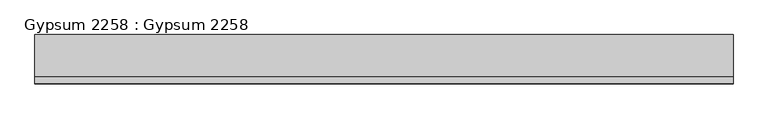
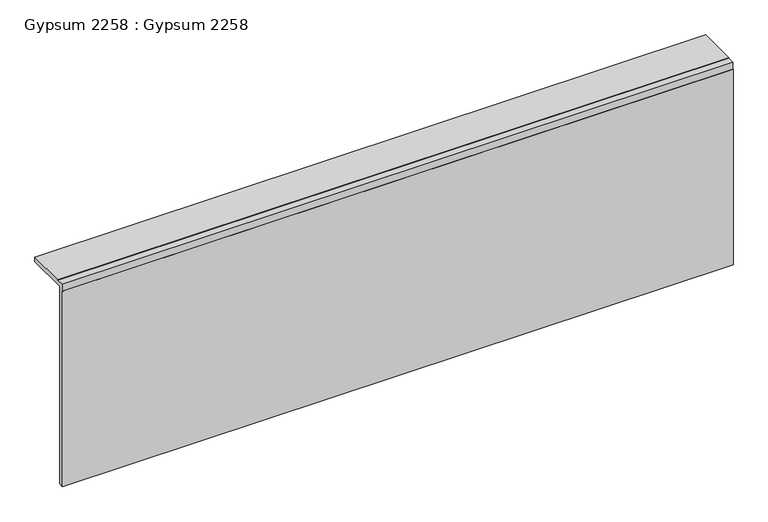
"""IFC4 building model written with IfcOpenShell, lengths in millimetres: proxy geometry, Gypsum 2258 : Gypsum 2258."""

from ifc_helpers import new_model, si_unit, frame, origin, place, context, project, spatial, polyline, outline, extrude, source, transform, mapped, element, save


def gypsum_2258_gypsum_2258_91d050d9(model_context):
    return source(origin(), model_context, "Body", "SweptSolid", [
        extrude(outline(polyline([(10263.7368438, 40772.8800973), (10265.0168438, 40772.8800973), (10265.0168438, 40794.0332812), (10286.1700277, 40794.0332812), (10286.1700277, 40795.3132812), (10405.3793386, 40795.3132812), (10405.3793386, 40779.84375), (10278.0250834, 40779.84375), (10278.0250834, 40157.1476563), (10263.7368438, 40157.1476563), (10263.7368438, 40772.8800973)])), frame((3694.2883192, 0.0, 0.0), z_axis=(1.0, 0.0, 0.0), x_axis=(0.0, 1.0, 0.0)), (0.0, 0.0, 1.0), 2000.0),
    ])


if __name__ == "__main__":
    model = new_model("IFC4")
    model_context = context("Model", 3, world=origin())
    ifc_project = project(units=[si_unit("LENGTHUNIT", "METRE", prefix="MILLI")], contexts=[model_context])
    site = spatial("IfcSite", under=ifc_project)
    building = spatial("IfcBuilding", under=site)
    placement = place(None, origin())
    gypsum_2258_gypsum_2258_shape = gypsum_2258_gypsum_2258_91d050d9(model_context)
    element("IfcBuildingElementProxy", 1, Name="Gypsum 2258 : Gypsum 2258", ObjectType="Gypsum 2258 : Gypsum 2258", at=placement, inside=building, context=model_context, shape_type="MappedRepresentation", body=[
        mapped(gypsum_2258_gypsum_2258_shape, transform((0.0, 0.0, 0.0), x_axis=(1.0, 0.0, 0.0), y_axis=(0.0, 1.0, 0.0), z_axis=(0.0, 0.0, 1.0))),
    ])
    save(model, "model.ifc")

# Revit data of these elements
# Type "Gypsum 2258 : Gypsum 2258"
#   NameOverride = "Gypsum"
# Element 1 (IfcBuildingElementProxy, "Gypsum 2258 : Gypsum 2258")
#   Materials on its faces: "5/8\"  GYPSUM BOARD"
# Materials
#   "5/8\"  GYPSUM BOARD": class "Unassigned", colour RGB 255 255 255, transparency 0, Cost = 0
